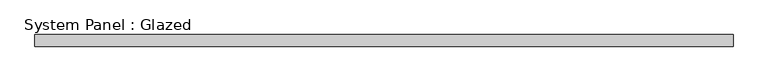
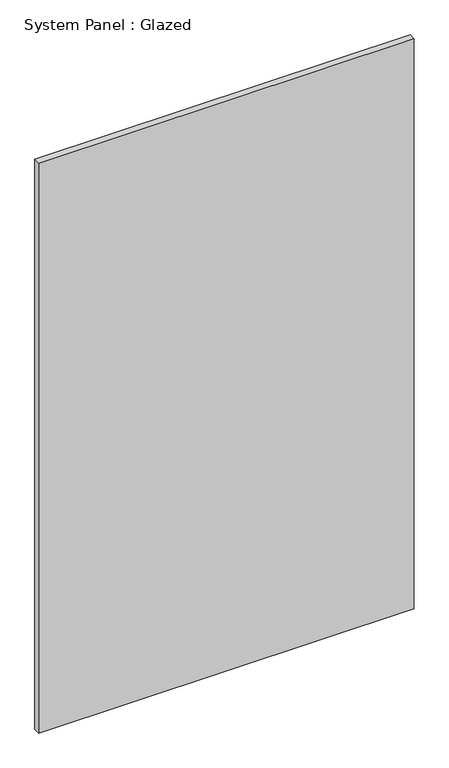
"""IFC4 building model written with IfcOpenShell, lengths in millimetres: plate geometry, System Panel : Glazed."""

from ifc_helpers import new_model, si_unit, origin, origin_with_axes, place, context, project, spatial, polyline, outline, extrude, source, transform, mapped, element, save


def system_panel_glazed_8d9daea7(model_context):
    return source(origin(), model_context, "Body", "SweptSolid", [
        extrude(outline(polyline([(724.9999999, 24.5), (-724.9999999, 24.5), (-724.9999999, 49.5), (724.9999999, 49.5), (724.9999999, 24.5)])), origin_with_axes(), (0.0, 0.0, 1.0), 2325.0),
    ])


if __name__ == "__main__":
    model = new_model("IFC4")
    model_context = context("Model", 3, world=origin())
    ifc_project = project(units=[si_unit("LENGTHUNIT", "METRE", prefix="MILLI")], contexts=[model_context])
    site = spatial("IfcSite", under=ifc_project)
    building = spatial("IfcBuilding", under=site)
    placement = place(None, origin())
    system_panel_glazed_shape = system_panel_glazed_8d9daea7(model_context)
    element("IfcPlate", 1, ObjectType="System Panel : Glazed", at=placement, inside=building, context=model_context, shape_type="MappedRepresentation", body=[
        mapped(system_panel_glazed_shape, transform((0.0, 0.0, 0.0), x_axis=(1.0, 0.0, 0.0), y_axis=(0.0, 1.0, 0.0), z_axis=(0.0, 0.0, 1.0))),
    ])
    save(model, "model.ifc")

# Revit data of these elements
# Type "System Panel : Glazed"
#   Construction Type Id = "GSP4R"
#   Analytic Construction = "1/8 in Pilkington single glazing"
#   Visual Light Transmittance = 0.9
#   Solar Heat Gain Coefficient = 0.86
#   Heat Transfer Coefficient (U) = 6.7069 W/(m²·K)
#   Define Thermal Properties by = 1
# Element 1 (IfcPlate, "System Panel : Glazed")
#   Materials on its faces: "Glass"
# Materials
#   "Glass": class "Glass", colour RGB 0 128 192, transparency 0.9, Description = "Soda Lime Glass", Cost = 0
